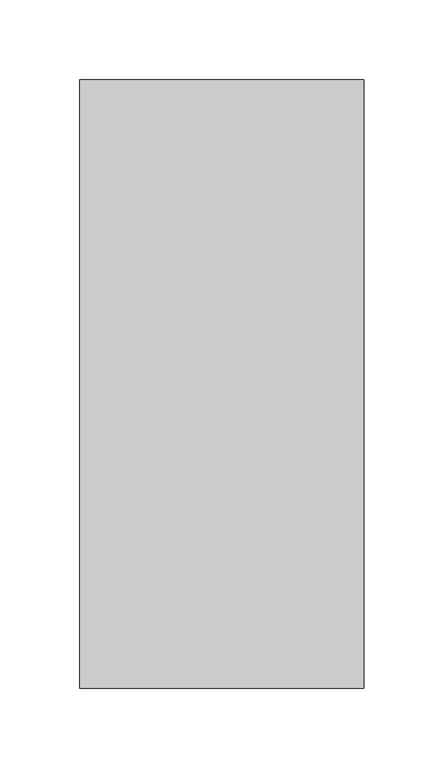
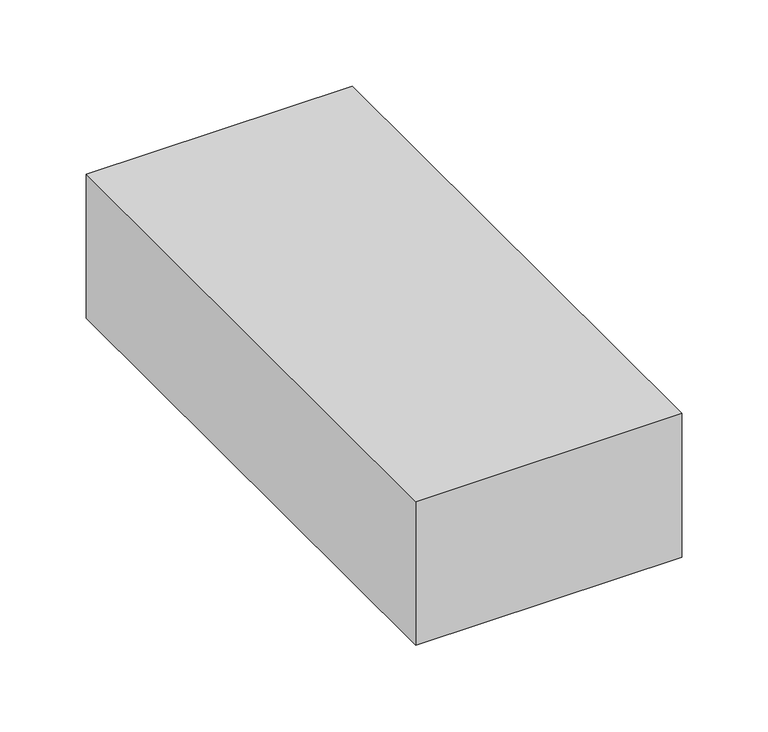
"""IFC4 building model written with IfcOpenShell, lengths in millimetres: proxy geometry, A5077 - Dispenser, Hand Sanitzer, Hands free : A5077 - Dispenser, Hand Sanitzer, Hands free."""

import ifcopenshell
import ifcopenshell.guid

model = None  # the IFC model being written
_history = None  # IfcOwnerHistory: only IFC2X3 demands one
_inside = {}  # id of a spatial element -> (the spatial element, [elements in it])
_under = {}  # id of a project, library or spatial element -> (it, [spatial elements below it])
_declared = {}  # id of a project -> (the project, [libraries it declares])
_typed = {}  # id of a type object -> (the type object, [elements of that type])
_made_of = {}  # id of a material, layer set ... -> (it, [elements and type objects made of it])


def new_model(schema):
    """Start an empty IFC model of exactly this schema.

    Asked for "IFC4X3", IfcOpenShell would pick the latest addendum, in which some entities
    have other attributes; the version numbers below select the first issue.
    IFC2X3 requires an IfcOwnerHistory on every rooted entity: one is made here for all.
    """
    global model, _history
    if schema == "IFC4X3":
        model = ifcopenshell.file(schema_version=(4, 3, 0, 0))
    else:
        model = ifcopenshell.file(schema=schema)
    _inside.clear()
    _under.clear()
    _declared.clear()
    _typed.clear()
    _made_of.clear()
    _history = None
    if model.schema == "IFC2X3":
        org = make("IfcOrganization", Name="unknown")
        user = make(
            "IfcPersonAndOrganization",
            ThePerson=make("IfcPerson", FamilyName="unknown"),
            TheOrganization=org,
        )
        app = make(
            "IfcApplication",
            ApplicationDeveloper=org,
            Version="unknown",
            ApplicationFullName="unknown",
            ApplicationIdentifier="unknown",
        )
        _history = make(
            "IfcOwnerHistory",
            OwningUser=user,
            OwningApplication=app,
            ChangeAction="ADDED",
            CreationDate=0,
        )
    return model


def make(cls, **values):
    """One entity of the class cls with the attributes given. An attribute that is None is left unset."""
    return model.create_entity(
        cls, **{name: value for name, value in values.items() if value is not None}
    )


def rooted(cls, **values):
    """An entity with a GlobalId (a new one), such as an element, a storey or a relation."""
    return make(cls, GlobalId=ifcopenshell.guid.new(), OwnerHistory=_history, **values)


def si_unit(unit_type, name, prefix=None):
    """IfcSIUnit, for example si_unit("LENGTHUNIT", "METRE", prefix="MILLI")."""
    return make("IfcSIUnit", UnitType=unit_type, Prefix=prefix, Name=name)


def assignment(units):
    """IfcUnitAssignment: the units of a project."""
    return None if units is None else make("IfcUnitAssignment", Units=units)


def point(xyz):
    """IfcCartesianPoint."""
    return None if xyz is None else make("IfcCartesianPoint", Coordinates=xyz)


def direction(xyz):
    """IfcDirection."""
    return None if xyz is None else make("IfcDirection", DirectionRatios=xyz)


def frame(location, z_axis=None, x_axis=None):
    """IfcAxis2Placement3D, a coordinate frame: its origin and axes. An axis left out is left unset."""
    return make(
        "IfcAxis2Placement3D",
        Location=point(location),
        Axis=direction(z_axis),
        RefDirection=direction(x_axis),
    )


def frame_2d(location, x_axis=None):
    """IfcAxis2Placement2D, a coordinate frame in the plane: its origin and x axis."""
    return make(
        "IfcAxis2Placement2D", Location=point(location), RefDirection=direction(x_axis)
    )


def origin():
    """The frame at (0, 0, 0) with its axes left unset."""
    return frame((0.0, 0.0, 0.0))


def origin_with_axes():
    """The frame at (0, 0, 0) with the z axis (0, 0, 1) and the x axis (1, 0, 0) written out."""
    return frame((0.0, 0.0, 0.0), z_axis=(0.0, 0.0, 1.0), x_axis=(1.0, 0.0, 0.0))


def place(relative_to, where):
    """IfcLocalPlacement: puts the frame where relative to a parent placement (None: the world)."""
    return make(
        "IfcLocalPlacement", PlacementRelTo=relative_to, RelativePlacement=where
    )


def context(
    kind, dimensions, precision=None, world=None, true_north=None, identifier=None
):
    """IfcGeometricRepresentationContext, for example the 3D "Model" context."""
    return make(
        "IfcGeometricRepresentationContext",
        ContextIdentifier=identifier,
        ContextType=kind,
        CoordinateSpaceDimension=dimensions,
        Precision=precision,
        WorldCoordinateSystem=world,
        TrueNorth=true_north,
    )


def project(units=None, contexts=None):
    """IfcProject with its units and contexts."""
    return rooted(
        "IfcProject",
        Name="project",
        RepresentationContexts=contexts,
        UnitsInContext=assignment(units),
    )


def spatial(cls, under=None, at=None, **own):
    """A site, building, storey or space (cls), placed at a placement, below another one or the project."""
    s = rooted(cls, ObjectPlacement=at, **own)
    if under is not None:
        _under.setdefault(under.id(), (under, []))[1].append(s)
    return s


def polyline(points):
    """IfcPolyline through the points."""
    return make("IfcPolyline", Points=[point(p) for p in points])


def circle_curve(where, radius):
    """IfcCircle in the frame where."""
    return make("IfcCircle", Position=where, Radius=radius)


def ellipse_curve(where, semi_axis1, semi_axis2):
    """IfcEllipse in the frame where."""
    return make(
        "IfcEllipse", Position=where, SemiAxis1=semi_axis1, SemiAxis2=semi_axis2
    )


def trimmed(basis, trim1, trim2, sense, master):
    """IfcTrimmedCurve: the piece of a basis curve between two trims."""
    return make(
        "IfcTrimmedCurve",
        BasisCurve=basis,
        Trim1=trim1,
        Trim2=trim2,
        SenseAgreement=sense,
        MasterRepresentation=master,
    )


def segment(curve, same_sense, transition):
    """IfcCompositeCurveSegment."""
    return make(
        "IfcCompositeCurveSegment",
        Transition=transition,
        SameSense=same_sense,
        ParentCurve=curve,
    )


def composite_curve(segments, self_intersect=None):
    """IfcCompositeCurve: segments joined end to end."""
    return make("IfcCompositeCurve", Segments=segments, SelfIntersect=self_intersect)


def outline(outer, holes=None, kind="AREA"):
    """IfcArbitraryClosedProfileDef: a profile drawn as a closed curve; with holes, ...WithVoids."""
    if holes is None:
        return make("IfcArbitraryClosedProfileDef", ProfileType=kind, OuterCurve=outer)
    return make(
        "IfcArbitraryProfileDefWithVoids",
        ProfileType=kind,
        OuterCurve=outer,
        InnerCurves=holes,
    )


def extrude(swept, where, along, depth):
    """IfcExtrudedAreaSolid: the profile swept, set in the frame where, extruded along a direction by depth."""
    return make(
        "IfcExtrudedAreaSolid",
        SweptArea=swept,
        Position=where,
        ExtrudedDirection=direction(along),
        Depth=depth,
    )


def shape(context_of_items, identifier, shape_type, items):
    """IfcShapeRepresentation: the items that make up one representation, for example the "Body"."""
    return make(
        "IfcShapeRepresentation",
        ContextOfItems=context_of_items,
        RepresentationIdentifier=identifier,
        RepresentationType=shape_type,
        Items=items,
    )


def source(mapping_origin, context_of_items, identifier, shape_type, items):
    """IfcRepresentationMap: a shape defined once, which mapped items show again and again."""
    return make(
        "IfcRepresentationMap",
        MappingOrigin=mapping_origin,
        MappedRepresentation=shape(context_of_items, identifier, shape_type, items),
    )


def transform(
    local_origin,
    x_axis=None,
    y_axis=None,
    z_axis=None,
    scale=None,
    scale2=None,
    scale3=None,
    uniform=True,
):
    """IfcCartesianTransformationOperator3D, or its non-uniform kind. x_axis, y_axis, z_axis: its Axis1, 2, 3."""
    if uniform:
        return make(
            "IfcCartesianTransformationOperator3D",
            Axis1=direction(x_axis),
            Axis2=direction(y_axis),
            LocalOrigin=point(local_origin),
            Scale=scale,
            Axis3=direction(z_axis),
        )
    return make(
        "IfcCartesianTransformationOperator3DnonUniform",
        Axis1=direction(x_axis),
        Axis2=direction(y_axis),
        LocalOrigin=point(local_origin),
        Scale=scale,
        Axis3=direction(z_axis),
        Scale2=scale2,
        Scale3=scale3,
    )


def mapped(mapping_source, mapping_target):
    """IfcMappedItem: shows the shape of a source again, moved by a transform."""
    return make(
        "IfcMappedItem", MappingSource=mapping_source, MappingTarget=mapping_target
    )


def made_of(thing, what):
    """Note that an element or type object is made of a material, layer set ...; save() writes the relation."""
    if what is not None:
        _made_of.setdefault(what.id(), (what, []))[1].append(thing)
    return thing


def element(
    cls,
    number,
    at=None,
    inside=None,
    cuts=None,
    type_object=None,
    material=None,
    context=None,
    identifier="Body",
    shape_type=None,
    held_by="IfcProductDefinitionShape",
    body=None,
    shapes=None,
    **own,
):
    """One element of the class cls, such as IfcWall. Its Tag is "e" and its number.

    at: its placement. inside: the storey or other place that contains it. cuts: it is an
    opening in that element (IfcRelVoidsElement). A single representation is given by context,
    identifier, shape_type and body (its items); several are given by shapes. held_by: the class
    of the entity that holds the representations. save() writes the other relations.
    """
    e = rooted(cls, Tag="e%d" % number, ObjectPlacement=at, **own)
    if body is not None:
        shapes = [shape(context, identifier, shape_type, body)]
    if shapes is not None:
        e.Representation = make(held_by, Representations=shapes)
    if inside is not None:
        _inside.setdefault(inside.id(), (inside, []))[1].append(e)
    if cuts is not None:
        rooted(
            "IfcRelVoidsElement", RelatingBuildingElement=cuts, RelatedOpeningElement=e
        )
    if type_object is not None:
        _typed.setdefault(type_object.id(), (type_object, []))[1].append(e)
    return made_of(e, material)


def aggregate(whole, parts):
    """IfcRelAggregates: a whole, such as a stair, and the parts it consists of."""
    return rooted("IfcRelAggregates", RelatingObject=whole, RelatedObjects=parts)


def save(model, path):
    """Write the relations noted so far, then the file.

    IfcRelAggregates (storeys below a building ...), IfcRelContainedInSpatialStructure (elements
    in a storey), IfcRelDefinesByType, IfcRelAssociatesMaterial and IfcRelDeclares: one each for
    every whole, place, type object, material and project.
    """
    for whole, parts in _under.values():
        aggregate(whole, parts)
    for where, things in _inside.values():
        rooted(
            "IfcRelContainedInSpatialStructure",
            RelatedElements=things,
            RelatingStructure=where,
        )
    for kind, things in _typed.values():
        rooted("IfcRelDefinesByType", RelatedObjects=things, RelatingType=kind)
    for what, things in _made_of.values():
        rooted("IfcRelAssociatesMaterial", RelatedObjects=things, RelatingMaterial=what)
    for by, libraries in _declared.values():
        rooted("IfcRelDeclares", RelatingContext=by, RelatedDefinitions=libraries)
    model.write(path)


def plane_surface(at):
    """IfcPlane: the flat surface through the origin of the frame at, square to its z axis."""
    return make("IfcPlane", Position=at)


def cylinder_surface(at, radius):
    """IfcCylindricalSurface: all points at the distance radius from the z axis of the frame at."""
    return make("IfcCylindricalSurface", Position=at, Radius=radius)


def revolved_surface(curve, axis_point, axis_direction):
    """IfcSurfaceOfRevolution: the curve turned about the line through axis_point along axis_direction."""
    return make(
        "IfcSurfaceOfRevolution",
        SweptCurve=make("IfcArbitraryOpenProfileDef", ProfileType="CURVE", Curve=curve),
        AxisPosition=make("IfcAxis1Placement", Location=point(axis_point), Axis=direction(axis_direction)),
    )


def advanced_brep(points, edges, surfaces, faces):
    """IfcAdvancedBrep: a solid bounded by faces that lie on surfaces and meet in shared edges.

    An edge is (start, end): straight between two places in points (the first is 0);
    or (start, end, curve); or (start, end, curve, False) where it runs against its curve.
    A face is (place in surfaces, loops), or (place, loops, False) where it looks against
    its surface's normal. A loop lists edges by number (the first is 1), with a minus sign
    where the edge is run from its end to its start. The first loop is the outer one.
    """
    corners = [point(p) for p in points]
    vertices = [make("IfcVertexPoint", VertexGeometry=c) for c in corners]
    made = []
    for start, end, *more in edges:
        made.append(
            make(
                "IfcEdgeCurve",
                EdgeStart=vertices[start],
                EdgeEnd=vertices[end],
                EdgeGeometry=more[0] if more else make("IfcPolyline", Points=[corners[start], corners[end]]),
                SameSense=more[1] if len(more) > 1 else True,
            )
        )
    hull = []
    for where, loops, *sense in faces:
        bounds = []
        for j, loop in enumerate(loops):
            ring = [make("IfcOrientedEdge", EdgeElement=made[abs(k) - 1], Orientation=k > 0) for k in loop]
            bounds.append(
                make(
                    "IfcFaceOuterBound" if j == 0 else "IfcFaceBound",
                    Bound=make("IfcEdgeLoop", EdgeList=ring),
                    Orientation=True,
                )
            )
        hull.append(make("IfcAdvancedFace", Bounds=bounds, FaceSurface=surfaces[where], SameSense=sense[0] if sense else True))
    return make("IfcAdvancedBrep", Outer=make("IfcClosedShell", CfsFaces=hull))


def specialty_equipment_af44a16f(model_context):
    return source(origin(), model_context, "Body", "SolidModel", [
        extrude(outline(composite_curve([segment(polyline([(-177.8, 57.15), (-176.2125, 57.15), (-176.2125, 7.14375)]), True, "CONTINUOUS"), segment(trimmed(circle_curve(frame_2d((-169.8625, 7.14375)), 6.35), [point((-176.2125, 7.14375))], [point((-169.8625, 0.79375))], True, "CARTESIAN"), True, "CONTINUOUS"), segment(polyline([(-169.8625, 0.79375), (-96.8375, 0.79375), (-96.8375, 0.0), (-177.8, 0.0), (-177.8, 57.15)]), True, "CONTINUOUS")], self_intersect=False)), frame((-73.025, 0.0, 0.0), z_axis=(1.0, 0.0, 0.0), x_axis=(0.0, 1.0, 0.0)), (0.0, 0.0, 1.0), 146.05),
        advanced_brep(
        [(-85.725, -85.725, 0.0), (-85.725, -28.575, 0.0), (-84.1375, -28.575, 0.0), (-84.1375, -85.725, 0.0), (-73.025, -96.8375, 0.0), (-73.025, -98.425, 0.0), (-85.725, -85.725, 50.8), (-85.725, -28.575, 50.8), (-66.675, -28.575, 69.85), (66.675, -28.575, 69.85), (85.725, -28.575, 50.8), (85.725, -28.575, 0.0), (84.1375, -28.575, 0.0), (84.1375, -28.575, 50.8), (66.675, -28.575, 68.2625), (-66.675, -28.575, 68.2625), (-84.1375, -28.575, 50.8), (-84.1375, -85.725, 50.8), (-73.025, -96.8375, 50.8), (-73.025, -98.425, 50.8), (-66.675, -85.725, 69.85), (-66.675, -85.725, 68.2625), (-66.675, -96.8375, 57.15), (-66.675, -98.425, 57.15), (66.675, -85.725, 69.85), (66.675, -85.725, 68.2625), (66.675, -96.8375, 57.15), (66.675, -98.425, 57.15), (85.725, -85.725, 50.8), (84.1375, -85.725, 50.8), (73.025, -96.8375, 50.8), (73.025, -98.425, 50.8), (85.725, -85.725, 0.0), (73.025, -98.425, 0.0), (73.025, -96.8375, 0.0), (84.1375, -85.725, 0.0)],
        [
            (0, 1),
            (1, 2),
            (2, 3),
            (3, 4, circle_curve(frame((-73.025, -85.725, 0.0), z_axis=(0.0, 0.0, 1.0), x_axis=(1.0, 0.0, 0.0)), 11.1125)),
            (4, 5),
            (5, 0, circle_curve(frame((-73.025, -85.725, 0.0), z_axis=(0.0, 0.0, -1.0), x_axis=(1.0, 0.0, 0.0)), 12.7)),
            (0, 6),
            (6, 7),
            (7, 1),
            (7, 8, circle_curve(frame((-66.675, -28.575, 50.8), z_axis=(0.0, 1.0, 0.0), x_axis=(-1.0, 0.0, 0.0)), 19.05)),
            (8, 9),
            (9, 10, circle_curve(frame((66.675, -28.575, 50.8), z_axis=(0.0, 1.0, 0.0), x_axis=(0.0, 0.0, 1.0)), 19.05)),
            (10, 11),
            (11, 12),
            (12, 13),
            (13, 14, circle_curve(frame((66.675, -28.575, 50.8), z_axis=(0.0, -1.0, 0.0), x_axis=(0.0, 0.0, 1.0)), 17.4625)),
            (14, 15),
            (15, 16, circle_curve(frame((-66.675, -28.575, 50.8), z_axis=(0.0, -1.0, 0.0), x_axis=(-1.0, 0.0, 0.0)), 17.4625)),
            (16, 2),
            (16, 17),
            (17, 3),
            (17, 18, circle_curve(frame((-73.025, -85.725, 50.8), z_axis=(0.0, 0.0, 1.0), x_axis=(1.0, 0.0, 0.0)), 11.1125)),
            (18, 4),
            (18, 19),
            (19, 5),
            (19, 6, circle_curve(frame((-73.025, -85.725, 50.8), z_axis=(0.0, 0.0, -1.0), x_axis=(1.0, 0.0, 0.0)), 12.7)),
            (6, 20, circle_curve(frame((-66.675, -85.725, 50.8), z_axis=(0.0, 1.0, 0.0), x_axis=(-1.0, 0.0, 0.0)), 19.05)),
            (20, 8),
            (21, 17, circle_curve(frame((-66.675, -85.725, 50.8), z_axis=(0.0, -1.0, 0.0), x_axis=(-1.0, 0.0, 0.0)), 17.4625)),
            (15, 21),
            (22, 18, circle_curve(frame((-66.675, -96.8375, 50.8), z_axis=(0.0, -1.0, 0.0), x_axis=(-1.0, 0.0, 0.0)), 6.35)),
            (21, 22, circle_curve(frame((-66.675, -85.725, 57.15), z_axis=(1.0, 0.0, 0.0), x_axis=(0.0, 0.0, -1.0)), 11.1125)),
            (23, 19, circle_curve(frame((-66.675, -98.425, 50.8), z_axis=(0.0, -1.0, 0.0), x_axis=(-1.0, 0.0, 0.0)), 6.35)),
            (22, 23),
            (23, 20, circle_curve(frame((-66.675, -85.725, 57.15), z_axis=(-1.0, 0.0, 0.0), x_axis=(0.0, 0.0, -1.0)), 12.7)),
            (20, 24),
            (24, 9),
            (14, 25),
            (25, 21),
            (25, 26, circle_curve(frame((66.675, -85.725, 57.15), z_axis=(1.0, 0.0, 0.0), x_axis=(0.0, 0.0, -1.0)), 11.1125)),
            (26, 22),
            (26, 27),
            (27, 23),
            (27, 24, circle_curve(frame((66.675, -85.725, 57.15), z_axis=(-1.0, 0.0, 0.0), x_axis=(0.0, 0.0, -1.0)), 12.7)),
            (24, 28, circle_curve(frame((66.675, -85.725, 50.8), z_axis=(0.0, 1.0, 0.0), x_axis=(0.0, 0.0, 1.0)), 19.05)),
            (28, 10),
            (29, 25, circle_curve(frame((66.675, -85.725, 50.8), z_axis=(0.0, -1.0, 0.0), x_axis=(0.0, 0.0, 1.0)), 17.4625)),
            (13, 29),
            (30, 26, circle_curve(frame((66.675, -96.8375, 50.8), z_axis=(0.0, -1.0, 0.0), x_axis=(0.0, 0.0, 1.0)), 6.35)),
            (29, 30, circle_curve(frame((73.025, -85.725, 50.8), z_axis=(0.0, 0.0, -1.0), x_axis=(-1.0, 0.0, 0.0)), 11.1125)),
            (31, 27, circle_curve(frame((66.675, -98.425, 50.8), z_axis=(0.0, -1.0, 0.0), x_axis=(0.0, 0.0, 1.0)), 6.35)),
            (30, 31),
            (31, 28, circle_curve(frame((73.025, -85.725, 50.8), z_axis=(0.0, 0.0, 1.0), x_axis=(-1.0, 0.0, 0.0)), 12.7)),
            (32, 33, circle_curve(frame((73.025, -85.725, 0.0), z_axis=(0.0, 0.0, -1.0), x_axis=(-1.0, 0.0, 0.0)), 12.7)),
            (33, 34),
            (34, 35, circle_curve(frame((73.025, -85.725, 0.0), z_axis=(0.0, 0.0, 1.0), x_axis=(-1.0, 0.0, 0.0)), 11.1125)),
            (35, 12),
            (11, 32),
            (28, 32),
            (35, 29),
            (34, 30),
            (33, 31),
        ],
        [
            plane_surface(frame((-85.725, -98.425, 0.0), z_axis=(0.0, 0.0, -1.0), x_axis=(0.0, 1.0, 0.0))),
            plane_surface(frame((-85.725, -85.725, 0.0), z_axis=(-1.0, 0.0, 0.0), x_axis=(0.0, 0.0, 1.0))),
            plane_surface(frame((-85.725, -28.575, 0.0), z_axis=(0.0, 1.0, 0.0), x_axis=(0.0, 0.0, 1.0))),
            plane_surface(frame((-84.1375, -28.575, 0.0), z_axis=(1.0, 0.0, 0.0), x_axis=(0.0, 0.0, 1.0))),
            revolved_surface(polyline([(-61.91250000000001, -85.725, 50.8), (-61.91250000000001, -85.725, 0.0)]), (-73.025, -85.725, 0.0), (0.0, 0.0, 1.0)),
            plane_surface(frame((-73.025, -96.8375, 0.0), z_axis=(1.0, 0.0, 0.0), x_axis=(0.0, 0.0, 1.0))),
            cylinder_surface(frame((-73.025, -85.725, 0.0), z_axis=(0.0, 0.0, -1.0), x_axis=(1.0, 0.0, 0.0)), 12.7),
            cylinder_surface(frame((-66.675, -98.425, 50.8), z_axis=(0.0, 1.0, 0.0), x_axis=(-1.0, 0.0, 0.0)), 19.05),
            revolved_surface(polyline([(-84.13749999999999, -28.575000000000003, 50.8), (-84.13749999999999, -85.725, 50.8)]), (-66.675, -98.425, 50.8), (0.0, 1.0, 0.0)),
            revolved_surface(trimmed(ellipse_curve(frame((-73.025, -85.725, 50.8), z_axis=(0.0, 0.0, 1.0), x_axis=(1.0, 0.0, 0.0)), 11.1125, 11.1125), [point((-84.1375, -85.725, 50.8))], [point((-73.025, -96.8375, 50.8))], True, "CARTESIAN"), (-66.675, -98.425, 50.8), (0.0, 1.0, 0.0)),
            revolved_surface(polyline([(-73.02499999999999, -96.8375, 50.8), (-73.02499999999999, -98.425, 50.8)]), (-66.675, -98.425, 50.8), (0.0, 1.0, 0.0)),
            revolved_surface(trimmed(ellipse_curve(frame((-73.025, -85.725, 50.8), z_axis=(0.0, 0.0, -1.0), x_axis=(1.0, 0.0, 0.0)), 12.7, 12.7), [point((-73.025, -98.425, 50.8))], [point((-85.725, -85.725, 50.8))], True, "CARTESIAN"), (-66.675, -98.425, 50.8), (0.0, 1.0, 0.0)),
            plane_surface(frame((-66.675, -85.725, 69.85), z_axis=(0.0, 0.0, 1.0), x_axis=(1.0, 0.0, 0.0))),
            plane_surface(frame((-66.675, -28.575, 68.2625), z_axis=(0.0, 0.0, -1.0), x_axis=(1.0, 0.0, 0.0))),
            revolved_surface(polyline([(66.675, -85.725, 46.037499999999994), (-66.675, -85.725, 46.037499999999994)]), (-66.675, -85.725, 57.15), (1.0, 0.0, 0.0)),
            plane_surface(frame((-66.675, -96.8375, 57.15), z_axis=(0.0, 0.0, -1.0), x_axis=(1.0, 0.0, 0.0))),
            cylinder_surface(frame((-66.675, -85.725, 57.15), z_axis=(-1.0, 0.0, 0.0), x_axis=(0.0, 0.0, -1.0)), 12.7),
            cylinder_surface(frame((66.675, -98.425, 50.8), z_axis=(0.0, 1.0, 0.0), x_axis=(0.0, 0.0, 1.0)), 19.05),
            revolved_surface(polyline([(66.675, -28.575000000000003, 68.26249999999999), (66.675, -85.725, 68.26249999999999)]), (66.675, -98.425, 50.8), (0.0, 1.0, 0.0)),
            revolved_surface(trimmed(ellipse_curve(frame((66.675, -85.725, 57.15), z_axis=(1.0, 0.0, 0.0), x_axis=(0.0, 0.0, -1.0)), 11.1125, 11.1125), [point((66.675, -85.725, 68.2625))], [point((66.675, -96.8375, 57.15))], True, "CARTESIAN"), (66.675, -98.425, 50.8), (0.0, 1.0, 0.0)),
            revolved_surface(polyline([(66.675, -96.8375, 57.15), (66.675, -98.425, 57.15)]), (66.675, -98.425, 50.8), (0.0, 1.0, 0.0)),
            revolved_surface(trimmed(ellipse_curve(frame((66.675, -85.725, 57.15), z_axis=(-1.0, 0.0, 0.0), x_axis=(0.0, 0.0, -1.0)), 12.7, 12.7), [point((66.675, -98.425, 57.15))], [point((66.675, -85.725, 69.85))], True, "CARTESIAN"), (66.675, -98.425, 50.8), (0.0, 1.0, 0.0)),
            plane_surface(frame((85.725, -98.425, 0.0), z_axis=(0.0, 0.0, -1.0), x_axis=(0.0, 1.0, 0.0))),
            plane_surface(frame((85.725, -85.725, 50.8), z_axis=(1.0, 0.0, 0.0), x_axis=(0.0, 0.0, -1.0))),
            plane_surface(frame((84.1375, -28.575, 50.8), z_axis=(-1.0, 0.0, 0.0), x_axis=(0.0, 0.0, -1.0))),
            revolved_surface(polyline([(61.91250000000001, -85.725, 0.0), (61.91250000000001, -85.725, 50.8)]), (73.025, -85.725, 50.8), (0.0, 0.0, -1.0)),
            plane_surface(frame((73.025, -96.8375, 50.8), z_axis=(-1.0, 0.0, 0.0), x_axis=(0.0, 0.0, -1.0))),
            cylinder_surface(frame((73.025, -85.725, 50.8), z_axis=(0.0, 0.0, 1.0), x_axis=(-1.0, 0.0, 0.0)), 12.7),
        ],
        [
            (0, [[1, 2, 3, 4, 5, 6]]),
            (1, [[-1, 7, 8, 9]]),
            (2, [[-2, -9, 10, 11, 12, 13, 14, 15, 16, 17, 18, 19]]),
            (3, [[-3, -19, 20, 21]]),
            (4, [[-4, -21, 22, 23]]),
            (5, [[-5, -23, 24, 25]]),
            (6, [[-6, -25, 26, -7]]),
            (7, [[-10, -8, 27, 28]]),
            (8, [[29, -20, -18, 30]]),
            (9, [[31, -22, -29, 32]]),
            (10, [[33, -24, -31, 34]]),
            (11, [[-27, -26, -33, 35]]),
            (12, [[-28, 36, 37, -11]]),
            (13, [[-30, -17, 38, 39]]),
            (14, [[-32, -39, 40, 41]]),
            (15, [[-34, -41, 42, 43]]),
            (16, [[-35, -43, 44, -36]]),
            (17, [[-12, -37, 45, 46]]),
            (18, [[47, -38, -16, 48]]),
            (19, [[49, -40, -47, 50]]),
            (20, [[51, -42, -49, 52]]),
            (21, [[-45, -44, -51, 53]]),
            (22, [[54, 55, 56, 57, -14, 58]]),
            (23, [[-46, 59, -58, -13]]),
            (24, [[-48, -15, -57, 60]]),
            (25, [[-50, -60, -56, 61]]),
            (26, [[-52, -61, -55, 62]]),
            (27, [[-53, -62, -54, -59]]),
        ],
    ),
        advanced_brep(
        [(-85.725, 165.1, 0.0), (-73.025, 177.8, 0.0), (-73.025, 176.2125, 0.0), (-84.1375, 165.1, 0.0), (-84.1375, 123.9305496, 0.0), (-85.725, 123.9305496, 0.0), (-85.725, 165.1, 50.8), (-73.025, 177.8, 50.8), (-73.025, 176.2125, 50.8), (-84.1375, 165.1, 50.8), (-84.1375, 123.9305496, 50.8), (-66.675, 123.9305496, 68.2625), (66.675, 123.9305496, 68.2625), (84.1375, 123.9305496, 50.8), (84.1375, 123.9305496, 0.0), (85.725, 123.9305496, 0.0), (85.725, 123.9305496, 50.8), (66.675, 123.9305496, 69.85), (-66.675, 123.9305496, 69.85), (-85.725, 123.9305496, 50.8), (-66.675, 177.8, 57.15), (-66.675, 165.1, 69.85), (-66.675, 176.2125, 57.15), (-66.675, 165.1, 68.2625), (66.675, 165.1, 69.85), (66.675, 177.8, 57.15), (66.675, 176.2125, 57.15), (66.675, 165.1, 68.2625), (73.025, 177.8, 50.8), (85.725, 165.1, 50.8), (73.025, 176.2125, 50.8), (84.1375, 165.1, 50.8), (85.725, 165.1, 0.0), (84.1375, 165.1, 0.0), (73.025, 176.2125, 0.0), (73.025, 177.8, 0.0)],
        [
            (0, 1, circle_curve(frame((-73.025, 165.1, 0.0), z_axis=(0.0, 0.0, -1.0), x_axis=(1.0, 0.0, 0.0)), 12.7)),
            (1, 2),
            (2, 3, circle_curve(frame((-73.025, 165.1, 0.0), z_axis=(0.0, 0.0, 1.0), x_axis=(1.0, 0.0, 0.0)), 11.1125)),
            (3, 4),
            (4, 5),
            (5, 0),
            (0, 6),
            (6, 7, circle_curve(frame((-73.025, 165.1, 50.8), z_axis=(0.0, 0.0, -1.0), x_axis=(1.0, 0.0, 0.0)), 12.7)),
            (7, 1),
            (7, 8),
            (8, 2),
            (8, 9, circle_curve(frame((-73.025, 165.1, 50.8), z_axis=(0.0, 0.0, 1.0), x_axis=(1.0, 0.0, 0.0)), 11.1125)),
            (9, 3),
            (9, 10),
            (10, 4),
            (10, 11, circle_curve(frame((-66.675, 123.9305496, 50.8), z_axis=(0.0, 1.0, 0.0), x_axis=(-1.0, 0.0, 0.0)), 17.4625)),
            (11, 12),
            (12, 13, circle_curve(frame((66.675, 123.9305496, 50.8), z_axis=(0.0, 1.0, 0.0), x_axis=(0.0, 0.0, 1.0)), 17.4625)),
            (13, 14),
            (14, 15),
            (15, 16),
            (16, 17, circle_curve(frame((66.675, 123.9305496, 50.8), z_axis=(0.0, -1.0, 0.0), x_axis=(0.0, 0.0, 1.0)), 19.05)),
            (17, 18),
            (18, 19, circle_curve(frame((-66.675, 123.9305496, 50.8), z_axis=(0.0, -1.0, 0.0), x_axis=(-1.0, 0.0, 0.0)), 19.05)),
            (19, 5),
            (19, 6),
            (20, 7, circle_curve(frame((-66.675, 177.8, 50.8), z_axis=(0.0, -1.0, 0.0), x_axis=(-1.0, 0.0, 0.0)), 6.35)),
            (6, 21, circle_curve(frame((-66.675, 165.1, 50.8), z_axis=(0.0, 1.0, 0.0), x_axis=(-1.0, 0.0, 0.0)), 19.05)),
            (21, 20, circle_curve(frame((-66.675, 165.1, 57.15), z_axis=(-1.0, 0.0, 0.0), x_axis=(0.0, 0.0, -1.0)), 12.7)),
            (22, 8, circle_curve(frame((-66.675, 176.2125, 50.8), z_axis=(0.0, -1.0, 0.0), x_axis=(-1.0, 0.0, 0.0)), 6.35)),
            (20, 22),
            (23, 9, circle_curve(frame((-66.675, 165.1, 50.8), z_axis=(0.0, -1.0, 0.0), x_axis=(-1.0, 0.0, 0.0)), 17.4625)),
            (22, 23, circle_curve(frame((-66.675, 165.1, 57.15), z_axis=(1.0, 0.0, 0.0), x_axis=(0.0, 0.0, -1.0)), 11.1125)),
            (23, 11),
            (18, 21),
            (21, 24),
            (24, 25, circle_curve(frame((66.675, 165.1, 57.15), z_axis=(-1.0, 0.0, 0.0), x_axis=(0.0, 0.0, -1.0)), 12.7)),
            (25, 20),
            (25, 26),
            (26, 22),
            (26, 27, circle_curve(frame((66.675, 165.1, 57.15), z_axis=(1.0, 0.0, 0.0), x_axis=(0.0, 0.0, -1.0)), 11.1125)),
            (27, 23),
            (27, 12),
            (17, 24),
            (28, 25, circle_curve(frame((66.675, 177.8, 50.8), z_axis=(0.0, -1.0, 0.0), x_axis=(0.0, 0.0, 1.0)), 6.35)),
            (24, 29, circle_curve(frame((66.675, 165.1, 50.8), z_axis=(0.0, 1.0, 0.0), x_axis=(0.0, 0.0, 1.0)), 19.05)),
            (29, 28, circle_curve(frame((73.025, 165.1, 50.8), z_axis=(0.0, 0.0, 1.0), x_axis=(-1.0, 0.0, 0.0)), 12.7)),
            (30, 26, circle_curve(frame((66.675, 176.2125, 50.8), z_axis=(0.0, -1.0, 0.0), x_axis=(0.0, 0.0, 1.0)), 6.35)),
            (28, 30),
            (31, 27, circle_curve(frame((66.675, 165.1, 50.8), z_axis=(0.0, -1.0, 0.0), x_axis=(0.0, 0.0, 1.0)), 17.4625)),
            (30, 31, circle_curve(frame((73.025, 165.1, 50.8), z_axis=(0.0, 0.0, -1.0), x_axis=(-1.0, 0.0, 0.0)), 11.1125)),
            (31, 13),
            (16, 29),
            (32, 15),
            (14, 33),
            (33, 34, circle_curve(frame((73.025, 165.1, 0.0), z_axis=(0.0, 0.0, 1.0), x_axis=(-1.0, 0.0, 0.0)), 11.1125)),
            (34, 35),
            (35, 32, circle_curve(frame((73.025, 165.1, 0.0), z_axis=(0.0, 0.0, -1.0), x_axis=(-1.0, 0.0, 0.0)), 12.7)),
            (29, 32),
            (35, 28),
            (34, 30),
            (33, 31),
        ],
        [
            plane_surface(frame((-85.725, 114.3, 0.0), z_axis=(0.0, 0.0, -1.0), x_axis=(0.0, 1.0, 0.0))),
            cylinder_surface(frame((-73.025, 165.1, 0.0), z_axis=(0.0, 0.0, -1.0), x_axis=(1.0, 0.0, 0.0)), 12.7),
            plane_surface(frame((-73.025, 177.8, 0.0), z_axis=(1.0, 0.0, 0.0), x_axis=(0.0, 0.0, 1.0))),
            revolved_surface(polyline([(-61.91250000000001, 165.1, 50.8), (-61.91250000000001, 165.1, 0.0)]), (-73.025, 165.1, 0.0), (0.0, 0.0, 1.0)),
            plane_surface(frame((-84.1375, 165.1, 0.0), z_axis=(1.0, 0.0, 0.0), x_axis=(0.0, 0.0, 1.0))),
            plane_surface(frame((-84.1375, 123.9305496, 0.0), z_axis=(0.0, -1.0, 0.0), x_axis=(0.0, 0.0, 1.0))),
            plane_surface(frame((-85.725, 123.9305496, 0.0), z_axis=(-1.0, 0.0, 0.0), x_axis=(0.0, 0.0, 1.0))),
            revolved_surface(trimmed(ellipse_curve(frame((-73.025, 165.1, 50.8), z_axis=(0.0, 0.0, -1.0), x_axis=(1.0, 0.0, 0.0)), 12.7, 12.7), [point((-85.725, 165.1, 50.8))], [point((-73.025, 177.8, 50.8))], True, "CARTESIAN"), (-66.675, 114.3, 50.8), (0.0, 1.0, 0.0)),
            revolved_surface(polyline([(-73.02499999999999, 177.8, 50.8), (-73.02499999999999, 176.2125, 50.8)]), (-66.675, 114.3, 50.8), (0.0, 1.0, 0.0)),
            revolved_surface(trimmed(ellipse_curve(frame((-73.025, 165.1, 50.8), z_axis=(0.0, 0.0, 1.0), x_axis=(1.0, 0.0, 0.0)), 11.1125, 11.1125), [point((-73.025, 176.2125, 50.8))], [point((-84.1375, 165.1, 50.8))], True, "CARTESIAN"), (-66.675, 114.3, 50.8), (0.0, 1.0, 0.0)),
            revolved_surface(polyline([(-84.13749999999999, 165.1, 50.8), (-84.13749999999999, 123.9305496, 50.8)]), (-66.675, 114.3, 50.8), (0.0, 1.0, 0.0)),
            cylinder_surface(frame((-66.675, 114.3, 50.8), z_axis=(0.0, 1.0, 0.0), x_axis=(-1.0, 0.0, 0.0)), 19.05),
            cylinder_surface(frame((-66.675, 165.1, 57.15), z_axis=(-1.0, 0.0, 0.0), x_axis=(0.0, 0.0, -1.0)), 12.7),
            plane_surface(frame((-66.675, 177.8, 57.15), z_axis=(0.0, 0.0, -1.0), x_axis=(1.0, 0.0, 0.0))),
            revolved_surface(polyline([(66.675, 165.1, 46.037499999999994), (-66.675, 165.1, 46.037499999999994)]), (-66.675, 165.1, 57.15), (1.0, 0.0, 0.0)),
            plane_surface(frame((-66.675, 165.1, 68.2625), z_axis=(0.0, 0.0, -1.0), x_axis=(1.0, 0.0, 0.0))),
            plane_surface(frame((-66.675, 123.9305496, 69.85), z_axis=(0.0, 0.0, 1.0), x_axis=(1.0, 0.0, 0.0))),
            revolved_surface(trimmed(ellipse_curve(frame((66.675, 165.1, 57.15), z_axis=(-1.0, 0.0, 0.0), x_axis=(0.0, 0.0, -1.0)), 12.7, 12.7), [point((66.675, 165.1, 69.85))], [point((66.675, 177.8, 57.15))], True, "CARTESIAN"), (66.675, 114.3, 50.8), (0.0, 1.0, 0.0)),
            revolved_surface(polyline([(66.675, 177.8, 57.15), (66.675, 176.2125, 57.15)]), (66.675, 114.3, 50.8), (0.0, 1.0, 0.0)),
            revolved_surface(trimmed(ellipse_curve(frame((66.675, 165.1, 57.15), z_axis=(1.0, 0.0, 0.0), x_axis=(0.0, 0.0, -1.0)), 11.1125, 11.1125), [point((66.675, 176.2125, 57.15))], [point((66.675, 165.1, 68.2625))], True, "CARTESIAN"), (66.675, 114.3, 50.8), (0.0, 1.0, 0.0)),
            revolved_surface(polyline([(66.675, 165.1, 68.26249999999999), (66.675, 123.9305496, 68.26249999999999)]), (66.675, 114.3, 50.8), (0.0, 1.0, 0.0)),
            cylinder_surface(frame((66.675, 114.3, 50.8), z_axis=(0.0, 1.0, 0.0), x_axis=(0.0, 0.0, 1.0)), 19.05),
            plane_surface(frame((85.725, 114.3, 0.0), z_axis=(0.0, 0.0, -1.0), x_axis=(0.0, 1.0, 0.0))),
            cylinder_surface(frame((73.025, 165.1, 50.8), z_axis=(0.0, 0.0, 1.0), x_axis=(-1.0, 0.0, 0.0)), 12.7),
            plane_surface(frame((73.025, 177.8, 50.8), z_axis=(-1.0, 0.0, 0.0), x_axis=(0.0, 0.0, -1.0))),
            revolved_surface(polyline([(61.91250000000001, 165.1, 0.0), (61.91250000000001, 165.1, 50.8)]), (73.025, 165.1, 50.8), (0.0, 0.0, -1.0)),
            plane_surface(frame((84.1375, 165.1, 50.8), z_axis=(-1.0, 0.0, 0.0), x_axis=(0.0, 0.0, -1.0))),
            plane_surface(frame((85.725, 123.9305496, 50.8), z_axis=(1.0, 0.0, 0.0), x_axis=(0.0, 0.0, -1.0))),
        ],
        [
            (0, [[1, 2, 3, 4, 5, 6]]),
            (1, [[-1, 7, 8, 9]]),
            (2, [[-2, -9, 10, 11]]),
            (3, [[-3, -11, 12, 13]]),
            (4, [[-4, -13, 14, 15]]),
            (5, [[-5, -15, 16, 17, 18, 19, 20, 21, 22, 23, 24, 25]]),
            (6, [[-6, -25, 26, -7]]),
            (7, [[27, -8, 28, 29]]),
            (8, [[30, -10, -27, 31]]),
            (9, [[32, -12, -30, 33]]),
            (10, [[-16, -14, -32, 34]]),
            (11, [[-28, -26, -24, 35]]),
            (12, [[-29, 36, 37, 38]]),
            (13, [[-31, -38, 39, 40]]),
            (14, [[-33, -40, 41, 42]]),
            (15, [[-34, -42, 43, -17]]),
            (16, [[-35, -23, 44, -36]]),
            (17, [[45, -37, 46, 47]]),
            (18, [[48, -39, -45, 49]]),
            (19, [[50, -41, -48, 51]]),
            (20, [[-18, -43, -50, 52]]),
            (21, [[-46, -44, -22, 53]]),
            (22, [[54, -20, 55, 56, 57, 58]]),
            (23, [[-47, 59, -58, 60]]),
            (24, [[-49, -60, -57, 61]]),
            (25, [[-51, -61, -56, 62]]),
            (26, [[-52, -62, -55, -19]]),
            (27, [[-53, -21, -54, -59]]),
        ],
    ),
        extrude(outline(composite_curve([segment(polyline([(50.8, -85.725), (0.0, -85.725), (0.0, -84.1375), (50.8, -84.1375)]), True, "CONTINUOUS"), segment(trimmed(circle_curve(frame_2d((50.8, -66.675)), 17.4625), [point((50.8, -84.1375))], [point((68.2625, -66.675))], True, "CARTESIAN"), True, "CONTINUOUS"), segment(polyline([(68.2625, -66.675), (68.2625, 66.675)]), True, "CONTINUOUS"), segment(trimmed(circle_curve(frame_2d((50.8, 66.675)), 17.4625), [point((68.2625, 66.675))], [point((50.8, 84.1375))], True, "CARTESIAN"), True, "CONTINUOUS"), segment(polyline([(50.8, 84.1375), (0.0, 84.1375), (0.0, 85.725), (50.8, 85.725)]), True, "CONTINUOUS"), segment(trimmed(circle_curve(frame_2d((50.8, 66.675)), 19.05), [point((50.8, 85.725))], [point((69.85, 66.675))], False, "CARTESIAN"), True, "CONTINUOUS"), segment(polyline([(69.85, 66.675), (69.85, -66.675)]), True, "CONTINUOUS"), segment(trimmed(circle_curve(frame_2d((50.8, -66.675)), 19.05), [point((69.85, -66.675))], [point((50.8, -85.725))], False, "CARTESIAN"), True, "CONTINUOUS")], self_intersect=False)), frame((0.0, -28.575, 0.0), z_axis=(0.0, 1.0, 0.0), x_axis=(0.0, 0.0, 1.0)), (0.0, 0.0, 1.0), 152.5055496),
        extrude(outline(composite_curve([segment(polyline([(68.2625, 66.675), (68.2625, -66.675)]), True, "CONTINUOUS"), segment(trimmed(circle_curve(frame_2d((50.8, -66.675)), 17.4625), [point((68.2625, -66.675))], [point((50.8, -84.1375))], False, "CARTESIAN"), True, "CONTINUOUS"), segment(polyline([(50.8, -84.1375), (0.0, -84.1375), (0.0, 84.1375), (50.8, 84.1375)]), True, "CONTINUOUS"), segment(trimmed(circle_curve(frame_2d((50.8, 66.675)), 17.4625), [point((50.8, 84.1375))], [point((68.2625, 66.675))], False, "CARTESIAN"), True, "CONTINUOUS")], self_intersect=False)), frame((0.0, -28.575, 0.0), z_axis=(0.0, 1.0, 0.0), x_axis=(0.0, 0.0, 1.0)), (0.0, 0.0, 1.0), 111.125),
        extrude(outline(composite_curve([segment(trimmed(circle_curve(frame_2d((41.275, 0.0)), 9.525), [point((41.275, -9.525))], [point((41.275, 9.525))], False, "CARTESIAN"), True, "CONTINUOUS"), segment(trimmed(circle_curve(frame_2d((41.275, 0.0)), 9.525), [point((41.275, 9.525))], [point((41.275, -9.525))], False, "CARTESIAN"), True, "CONTINUOUS")], self_intersect=False)), frame((0.0, -111.125, 0.0), z_axis=(0.0, 1.0, 0.0), x_axis=(0.0, 0.0, 1.0)), (0.0, 0.0, 1.0), 12.7),
        extrude(outline(composite_curve([segment(polyline([(0.0, -73.025), (0.0, 73.025), (50.8, 73.025)]), True, "CONTINUOUS"), segment(trimmed(circle_curve(frame_2d((50.8, 66.675)), 6.35), [point((50.8, 73.025))], [point((57.15, 66.675))], False, "CARTESIAN"), True, "CONTINUOUS"), segment(polyline([(57.15, 66.675), (57.15, -66.675)]), True, "CONTINUOUS"), segment(trimmed(circle_curve(frame_2d((50.8, -66.675)), 6.35), [point((57.15, -66.675))], [point((50.8, -73.025))], False, "CARTESIAN"), True, "CONTINUOUS"), segment(polyline([(50.8, -73.025), (0.0, -73.025)]), True, "CONTINUOUS")], self_intersect=False)), frame((0.0, -98.425, 0.0), z_axis=(0.0, 1.0, 0.0), x_axis=(0.0, 0.0, 1.0)), (0.0, 0.0, 1.0), 1.5875),
        extrude(outline(polyline([(88.9, 190.5), (88.9, -190.5), (-88.9, -190.5), (-88.9, 190.5), (88.9, 190.5)])), origin_with_axes(), (0.0, 0.0, 1.0), 101.6),
        extrude(outline(composite_curve([segment(polyline([(0.0, -73.025), (0.0, 73.025), (50.8, 73.025)]), True, "CONTINUOUS"), segment(trimmed(circle_curve(frame_2d((50.8, 66.675)), 6.35), [point((50.8, 73.025))], [point((57.15, 66.675))], False, "CARTESIAN"), True, "CONTINUOUS"), segment(polyline([(57.15, 66.675), (57.15, -66.675)]), True, "CONTINUOUS"), segment(trimmed(circle_curve(frame_2d((50.8, -66.675)), 6.35), [point((57.15, -66.675))], [point((50.8, -73.025))], False, "CARTESIAN"), True, "CONTINUOUS"), segment(polyline([(50.8, -73.025), (0.0, -73.025)]), True, "CONTINUOUS")], self_intersect=False)), frame((0.0, 176.2125, 0.0), z_axis=(0.0, 1.0, 0.0), x_axis=(0.0, 0.0, 1.0)), (0.0, 0.0, 1.0), 1.5875),
    ])


if __name__ == "__main__":
    model = new_model("IFC4")
    model_context = context("Model", 3, world=origin())
    ifc_project = project(units=[si_unit("LENGTHUNIT", "METRE", prefix="MILLI")], contexts=[model_context])
    site = spatial("IfcSite", under=ifc_project)
    building = spatial("IfcBuilding", under=site)
    placement = place(None, origin())
    specialty_equipment_shape = specialty_equipment_af44a16f(model_context)
    element("IfcBuildingElementProxy", 1, Name="A5077 - Dispenser, Hand Sanitzer, Hands free : A5077 - Dispenser, Hand Sanitzer, Hands free", ObjectType="A5077 - Dispenser, Hand Sanitzer, Hands free : A5077 - Dispenser, Hand Sanitzer, Hands free", at=placement, inside=building, context=model_context, shape_type="MappedRepresentation", body=[
        mapped(specialty_equipment_shape, transform((0.0, 0.0, 0.0), x_axis=(1.0, 0.0, 0.0), y_axis=(0.0, 1.0, 0.0), z_axis=(0.0, 0.0, 1.0))),
    ])
    save(model, "model.ifc")

# Revit data of these elements
# Type "A5077 - Dispenser, Hand Sanitzer, Hands free : A5077 - Dispenser, Hand Sanitzer, Hands free"
#   Watts2 = "0"
#   Watts1 = "0"
#   Unit_Issue = "EA"
#   UTIL_6_Misc = "-"
#   UTIL_5_NonMedGas = "-"
#   UTIL_4_MiscGas = "-"
#   UTIL_3_MedGas = "-"
#   UTIL_2_Elec = "-"
#   UTIL_1_WaterDrain = "-"
#   Nomenclature = "Dispenser, Hand Sanitzer, Hands free"
#   NSN = ""
#   Location [instance default] = ""
#   JSN = "A5077"
#   Fund_Source_VA = "-"
#   Fund_Source_Navy = "-"
#   Fund_Source_Army = "-"
#   Fund_Source_AF = "-"
#   ELEC_Volts2 = "0"
#   ELEC_Volts1 = "0"
#   ELEC_Phase2 = "0"
#   ELEC_Phase1 = "0"
#   ELEC_HertzSwitch = "0"
#   ELEC_HertzDependent = "0"
#   ELEC_Hertz = "0"
#   ELEC_Amps2 = "0"
#   ELEC_Amps1 = "0"
#   DetailDescription = ""
#   CAT_VA = "C"
#   CAT_Navy = "C"
#   CAT_IHS = "-"
#   CAT_Army = "C"
#   CAT_AF = "C"
#   BTUperhour = "0"
#   Weight_IP = 0
#   Default Elevation = 4' - 0"
#   DIM_Width_IP = 0' - 7"
#   DIM_Height_IP = 1' - 3"
#   DIM_Depth_IP = 0' - 6"
# Element 1 (IfcBuildingElementProxy, "A5077 - Dispenser, Hand Sanitzer, Hands free : A5077 - Dispenser, Hand Sanitzer, Hands free")
#   Materials on its faces: "White Paint", "Glass", "EquipSpace"
# Materials
#   "White Paint": class "Unassigned", colour RGB 249 249 249, transparency 0
#   "Glass": class "Glass", colour RGB 0 128 192, transparency 0.75
#   "EquipSpace": class "Unassigned", colour RGB 221 217 195, transparency 0.5
